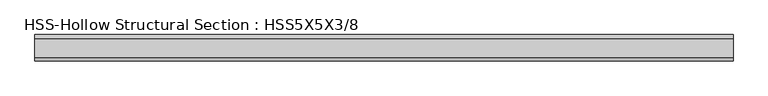
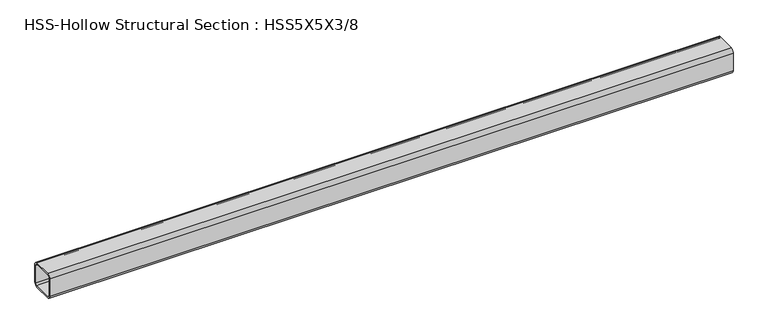
"""IFC4 building model written with IfcOpenShell, lengths in millimetres: member geometry, HSS-Hollow Structural Section : HSS5X5X3/8."""

from ifc_helpers import new_model, si_unit, point, frame, frame_2d, origin, place, context, project, spatial, polyline, circle_curve, trimmed, segment, composite_curve, outline, extrude, source, transform, mapped, element, save


def hss_hollow_structural_section_hss5x5x3_8_d5127346(model_context):
    return source(origin(), model_context, "Body", "SweptSolid", [
        extrude(outline(composite_curve([segment(polyline([(63.5, 45.7708), (63.5, -45.7708)]), True, "CONTINUOUS"), segment(trimmed(circle_curve(frame_2d((45.7708, -45.7708)), 17.7292), [point((63.5, -45.7708))], [point((45.7708, -63.5))], False, "CARTESIAN"), True, "CONTINUOUS"), segment(polyline([(45.7708, -63.5), (-45.7708, -63.5)]), True, "CONTINUOUS"), segment(trimmed(circle_curve(frame_2d((-45.7708, -45.7708)), 17.7292), [point((-45.7708, -63.5))], [point((-63.5, -45.7708))], False, "CARTESIAN"), True, "CONTINUOUS"), segment(polyline([(-63.5, -45.7708), (-63.5, 45.7708)]), True, "CONTINUOUS"), segment(trimmed(circle_curve(frame_2d((-45.7708, 45.7708)), 17.7292), [point((-63.5, 45.7708))], [point((-45.7708, 63.5))], False, "CARTESIAN"), True, "CONTINUOUS"), segment(polyline([(-45.7708, 63.5), (45.7708, 63.5)]), True, "CONTINUOUS"), segment(trimmed(circle_curve(frame_2d((45.7708, 45.7708)), 17.7292), [point((45.7708, 63.5))], [point((63.5, 45.7708))], False, "CARTESIAN"), True, "CONTINUOUS")], self_intersect=False), holes=[composite_curve([segment(trimmed(circle_curve(frame_2d((-45.7708, 45.7708)), 8.8646), [point((-45.7708, 54.6354))], [point((-54.6354, 45.7708))], True, "CARTESIAN"), True, "CONTINUOUS"), segment(polyline([(-54.6354, 45.7708), (-54.6354, -45.7708)]), True, "CONTINUOUS"), segment(trimmed(circle_curve(frame_2d((-45.7708, -45.7708)), 8.8646), [point((-54.6354, -45.7708))], [point((-45.7708, -54.6354))], True, "CARTESIAN"), True, "CONTINUOUS"), segment(polyline([(-45.7708, -54.6354), (45.7708, -54.6354)]), True, "CONTINUOUS"), segment(trimmed(circle_curve(frame_2d((45.7708, -45.7708)), 8.8646), [point((45.7708, -54.6354))], [point((54.6354, -45.7708))], True, "CARTESIAN"), True, "CONTINUOUS"), segment(polyline([(54.6354, -45.7708), (54.6354, 45.7708)]), True, "CONTINUOUS"), segment(trimmed(circle_curve(frame_2d((45.7708, 45.7708)), 8.8646), [point((54.6354, 45.7708))], [point((45.7708, 54.6354))], True, "CARTESIAN"), True, "CONTINUOUS"), segment(polyline([(45.7708, 54.6354), (-45.7708, 54.6354)]), True, "CONTINUOUS")], self_intersect=False)]), frame((-1649.8052265, 0.0, 0.0), z_axis=(1.0, 0.0, 0.0), x_axis=(0.0, 1.0, 0.0)), (0.0, 0.0, 1.0), 3369.6564507),
    ])


if __name__ == "__main__":
    model = new_model("IFC4")
    model_context = context("Model", 3, world=origin())
    ifc_project = project(units=[si_unit("LENGTHUNIT", "METRE", prefix="MILLI")], contexts=[model_context])
    site = spatial("IfcSite", under=ifc_project)
    building = spatial("IfcBuilding", under=site)
    placement = place(None, origin())
    hss_hollow_structural_section_hss5x5x3_8_shape = hss_hollow_structural_section_hss5x5x3_8_d5127346(model_context)
    element("IfcMember", 1, ObjectType="HSS-Hollow Structural Section : HSS5X5X3/8", at=placement, inside=building, context=model_context, shape_type="MappedRepresentation", body=[
        mapped(hss_hollow_structural_section_hss5x5x3_8_shape, transform((0.0, 0.0, 0.0), x_axis=(1.0, 0.0, 0.0), y_axis=(0.0, 1.0, 0.0), z_axis=(0.0, 0.0, 1.0))),
    ])
    save(model, "model.ifc")

# Revit data of these elements
# Type "HSS-Hollow Structural Section : HSS5X5X3/8"
#   Assembly Code = "B10"
#   Shape = "Square"
#   W = 22.3
#   Ht = 0' - 5"
#   Length [instance default] = 5' - 0"
#   b = 0' - 5"
#   kr = 0' - 0.698"
#   t = 0' - 0.349"
#   A = 0.0429167 SF
#   Structural Material [instance default] = Steel ASTM A500, Grade B, Rectangular and Square
# Element 1 (IfcMember, "HSS-Hollow Structural Section : HSS5X5X3/8")
#   Materials on its faces: "Steel ASTM A500, Grade B, Rectangular and Square"
# Materials
#   "Steel ASTM A500, Grade B, Rectangular and Square": class "Metal", colour RGB 199 199 199, transparency 0, Description = "Carbon steel", Cost = 0
